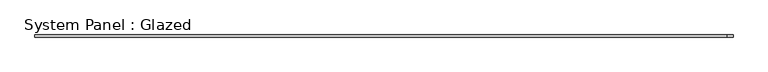
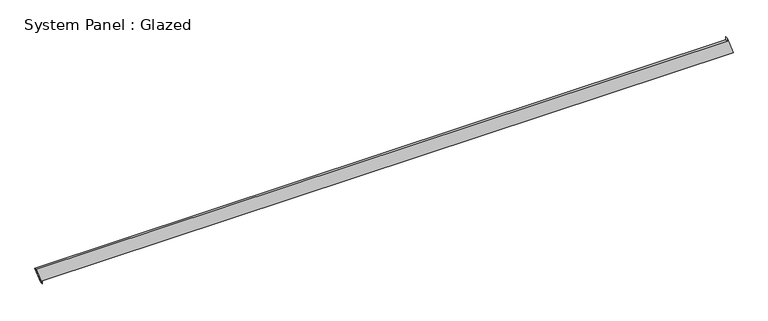
"""IFC4 building model written with IfcOpenShell, lengths in millimetres: plate geometry, System Panel : Glazed."""

from ifc_helpers import new_model, si_unit, frame, origin, place, context, project, spatial, polyline, outline, extrude, source, transform, mapped, element, save


def system_panel_glazed_3920cfb5(model_context):
    return source(origin(), model_context, "Body", "SweptSolid", [
        extrude(outline(polyline([(0.0, -3957.1612499), (35.3553391, -3957.1612499), (35.3553391, 4027.0933919), (235.3468796, 3957.4323455), (199.9915406, 3957.4328486), (199.8779154, -4027.0933919), (0.0, -3957.1612499)])), frame((0.0, -49.5, 0.0), z_axis=(0.0, 1.0, 0.0), x_axis=(0.0, 0.0, 1.0)), (0.0, 0.0, 1.0), 25.0),
    ])


if __name__ == "__main__":
    model = new_model("IFC4")
    model_context = context("Model", 3, world=origin())
    ifc_project = project(units=[si_unit("LENGTHUNIT", "METRE", prefix="MILLI")], contexts=[model_context])
    site = spatial("IfcSite", under=ifc_project)
    building = spatial("IfcBuilding", under=site)
    placement = place(None, origin())
    system_panel_glazed_shape = system_panel_glazed_3920cfb5(model_context)
    element("IfcPlate", 1, ObjectType="System Panel : Glazed", at=placement, inside=building, context=model_context, shape_type="MappedRepresentation", body=[
        mapped(system_panel_glazed_shape, transform((0.0, 0.0, 0.0), x_axis=(1.0, 0.0, 0.0), y_axis=(0.0, 1.0, 0.0), z_axis=(0.0, 0.0, 1.0))),
    ])
    save(model, "model.ifc")

# Revit data of these elements
# Element 1 (IfcPlate, "System Panel : Glazed")
#   Materials on its faces: "Glass"
# Materials
#   "Glass": class "Glass", colour RGB 218 227 224, transparency 0.85, Description = "Soda Lime Glass", Cost = 0
